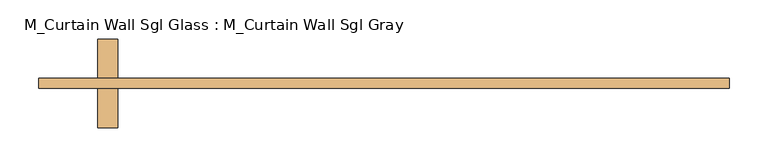
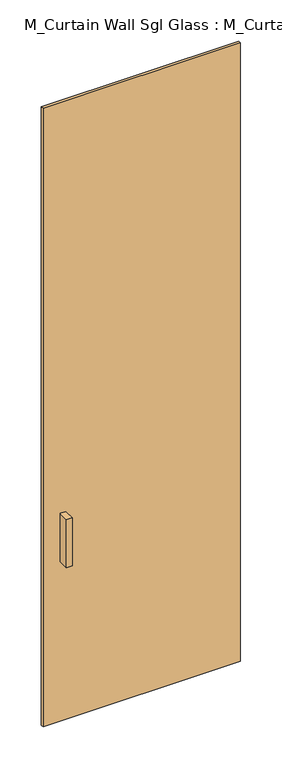
"""IFC4 building model written with IfcOpenShell, lengths in millimetres: door geometry, M_Curtain Wall Sgl Glass : M_Curtain Wall Sgl Gray."""

from ifc_helpers import new_model, si_unit, frame, origin, origin_with_axes, place, context, project, spatial, polyline, outline, extrude, source, transform, mapped, element, save


def m_curtain_wall_sgl_glass_m_curtain_wall_sgl_gray_5ebf1b51(model_context):
    return source(origin(), model_context, "Body", "SweptSolid", [
        extrude(outline(polyline([(-343.4, 12.5), (-343.4, -38.3), (-368.8, -38.3), (-368.8, 12.5), (-343.4, 12.5)])), frame((0.0, 0.0, 762.0), z_axis=(0.0, 0.0, 1.0), x_axis=(1.0, 0.0, 0.0)), (0.0, 0.0, 1.0), 228.6),
        extrude(outline(polyline([(-368.8, -101.8), (-368.8, -51.0), (-343.4, -51.0), (-343.4, -101.8), (-368.8, -101.8)])), frame((0.0, 0.0, 762.0), z_axis=(0.0, 0.0, 1.0), x_axis=(1.0, 0.0, 0.0)), (0.0, 0.0, 1.0), 228.6),
        extrude(outline(polyline([(445.0, -51.0), (-445.0, -51.0), (-445.0, -38.3), (445.0, -38.3), (445.0, -51.0)])), origin_with_axes(), (0.0, 0.0, 1.0), 2950.0),
    ])


if __name__ == "__main__":
    model = new_model("IFC4")
    model_context = context("Model", 3, world=origin())
    ifc_project = project(units=[si_unit("LENGTHUNIT", "METRE", prefix="MILLI")], contexts=[model_context])
    site = spatial("IfcSite", under=ifc_project)
    building = spatial("IfcBuilding", under=site)
    placement = place(None, origin())
    m_curtain_wall_sgl_glass_m_curtain_wall_sgl_gray_shape = m_curtain_wall_sgl_glass_m_curtain_wall_sgl_gray_5ebf1b51(model_context)
    element("IfcDoor", 1, ObjectType="M_Curtain Wall Sgl Glass : M_Curtain Wall Sgl Gray", at=placement, inside=building, context=model_context, shape_type="MappedRepresentation", body=[
        mapped(m_curtain_wall_sgl_glass_m_curtain_wall_sgl_gray_shape, transform((0.0, 0.0, 0.0), x_axis=(1.0, 0.0, 0.0), y_axis=(0.0, 1.0, 0.0), z_axis=(0.0, 0.0, 1.0))),
    ])
    save(model, "model.ifc")

# Revit data of these elements
# Type "M_Curtain Wall Sgl Glass : M_Curtain Wall Sgl Gray"
#   Model = "12345667"
#   Manufacturer = "Dublin Doors"
#   Description = "Single Flush door"
#   Type Mark = "48"
#   COBie.Type.CreatedBy = "design@eagle.com"
#   COBie.Type.CreatedOn = "2016-09-13T05:47:35"
#   COBie.Type.Name = "Doors_M_Curtain Wall Sgl Glass_M_Curtain Wall Sgl Gray"
#   COBie.Type.Category = "23-30 10 00 : Doors"
#   COBie.Type.Description = "Single Flush door"
#   COBie.Type.Manufacturer = "Dublin Doors"
#   COBie.Type.ModelNumber = "12345667"
#   Construction Type Id = "opn-d36"
#   Analytic Construction = "Wood panel"
#   COBie.Type.ReplacementCost = 0
#   Offset = 51 mm
#   Heat Transfer Coefficient (U) = 3.8042 W/(m²·K)
#   COBie.Type = yes
#   Function = 1
#   Glazing Material = Door - Frame(1)
#   Visual Light Transmittance = 0
#   Solar Heat Gain Coefficient = 0
# Element 1 (IfcDoor, "M_Curtain Wall Sgl Glass : M_Curtain Wall Sgl Gray")
#   Materials on its faces: "Aluminum", "Door - Frame(1)"
# Materials
#   "Door - Frame(1)": class "Miscellaneous", colour RGB 128 128 128, transparency 0, Cost = 0
#   "Aluminum": class "Metal", colour RGB 247 247 247, transparency 0, Description = "Aluminum 6061", Cost = 0
